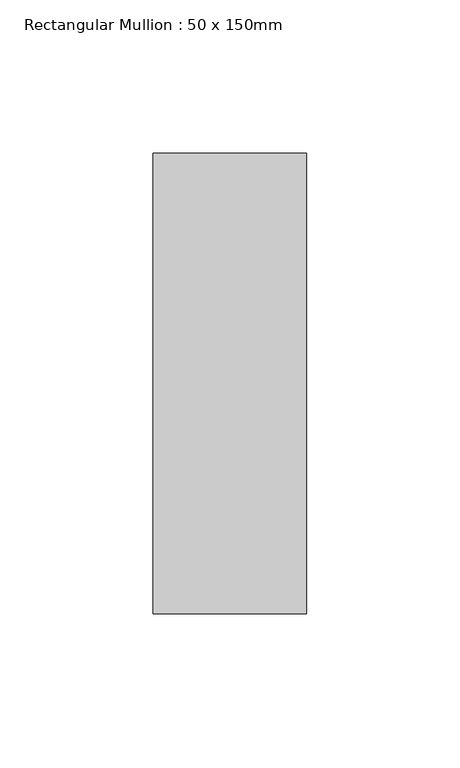
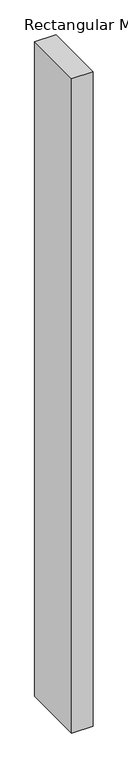
"""IFC4 building model written with IfcOpenShell, lengths in millimetres: member geometry, Rectangular Mullion : 50 x 150mm."""

from ifc_helpers import new_model, si_unit, frame, origin, place, context, project, spatial, polyline, outline, extrude, source, transform, mapped, element, save


def rectangular_mullion_50_x_150mm_a561114d(model_context):
    return source(origin(), model_context, "Body", "SweptSolid", [
        extrude(outline(polyline([(25.0, 75.0), (25.0, -75.0), (-25.0, -75.0), (-25.0, 75.0), (25.0, 75.0)])), frame((0.0, 0.0, -1615.55), z_axis=(0.0, 0.0, 1.0), x_axis=(1.0, 0.0, 0.0)), (0.0, 0.0, 1.0), 1615.55),
    ])


if __name__ == "__main__":
    model = new_model("IFC4")
    model_context = context("Model", 3, world=origin())
    ifc_project = project(units=[si_unit("LENGTHUNIT", "METRE", prefix="MILLI")], contexts=[model_context])
    site = spatial("IfcSite", under=ifc_project)
    building = spatial("IfcBuilding", under=site)
    placement = place(None, origin())
    rectangular_mullion_50_x_150mm_shape = rectangular_mullion_50_x_150mm_a561114d(model_context)
    element("IfcMember", 1, ObjectType="Rectangular Mullion : 50 x 150mm", at=placement, inside=building, context=model_context, shape_type="MappedRepresentation", body=[
        mapped(rectangular_mullion_50_x_150mm_shape, transform((0.0, 0.0, 0.0), x_axis=(1.0, 0.0, 0.0), y_axis=(0.0, 1.0, 0.0), z_axis=(0.0, 0.0, 1.0))),
    ])
    save(model, "model.ifc")

# Revit data of these elements
# Type "Rectangular Mullion : 50 x 150mm"
#   Keynote = "H11"
#   built-in parameter 1007304 = 0.492126 (stored number, unit not read)
#   built-in parameter 1007301 = 0.082021 (stored number, unit not read)
#   built-in parameter 1007300 = 0.082021 (stored number, unit not read)
# Element 1 (IfcMember, "Rectangular Mullion : 50 x 150mm")
#   Materials on its faces: "Aluminium"
# Materials
#   "Aluminium": class "Metal", colour RGB 247 247 247, transparency 0, Description = "Aluminium 6061", Cost = 0
